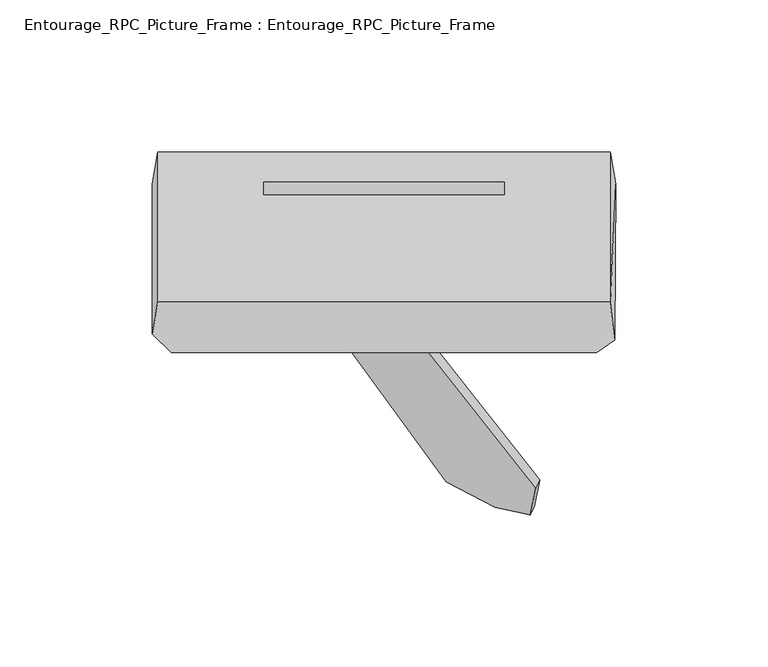
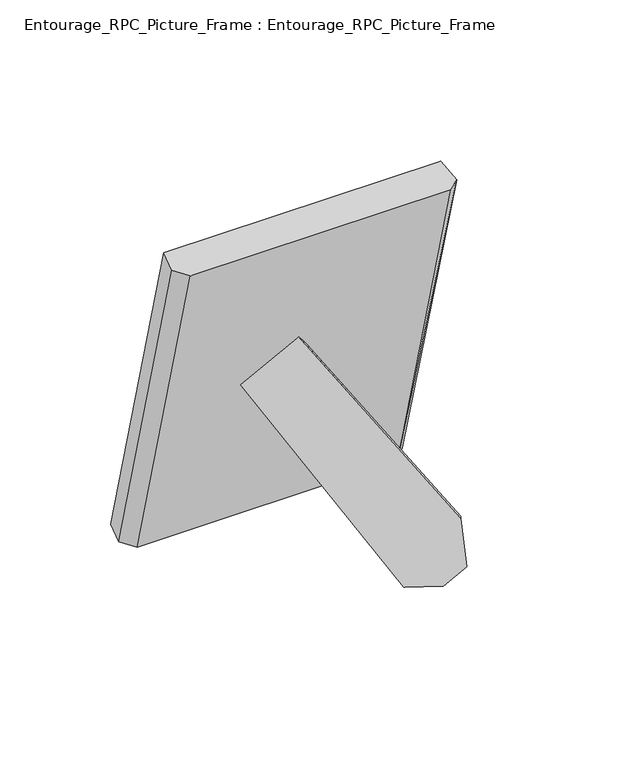
"""IFC4 building model written with IfcOpenShell, lengths in millimetres: proxy geometry, Entourage_RPC_Picture_Frame : Entourage_RPC_Picture_Frame."""

from ifc_helpers import new_model, si_unit, origin, place, context, project, spatial, triangles, source, transform, mapped, element, save


def entourage_rpc_picture_frame_entourage_rpc_picture_frame_0c3f382a(model_context):
    return source(origin(), model_context, "Body", "Tessellation", [
        triangles([(-31.2212752, 21.3179439, 97.8039775), (-3.3552966, 15.6563572, 118.0830721), (49.8722556, -51.6400711, 31.432093), (48.0637995, -60.4893174, 9.6569551), (36.5907671, -58.1576284, 1.3080831), (20.4721357, -49.6588966, 1.1709248), (-29.8344526, 23.9264897, 96.6279682), (-1.9710145, 18.262363, 116.9070629), (51.2565371, -49.0391442, 30.2611684), (49.4455375, -57.8858517, 8.4834904), (37.9725073, -55.5541626, 0.1346183), (21.8564171, -47.0554308, -0.00254), (-74.3118158, 9.430898, 188.4655675), (74.3118158, 9.430898, 188.4655675), (75.7926166, -3.1317793, 185.1001116), (69.8490931, -7.2160464, 184.0053746), (-69.8490931, -7.2160464, 184.0053746), (-76.1990144, -1.082026, 185.6487336), (-74.3118158, 58.7342011, 4.4601824), (74.3118158, 58.7469002, 4.4398626), (76.1990144, 48.2212754, 1.6433587), (69.8490931, 42.0897955, 0.0), (-69.8490931, 42.0897955, 0.0), (-76.1990144, 48.2212754, 1.6433587), (-39.6869853, 19.0954732, 152.4335917), (39.6869853, 19.0954732, 152.436117), (39.6869853, 49.0899451, 40.4972374), (-39.6869853, 49.0899451, 40.4972374), (-39.6869853, 14.7064095, 151.2575824), (39.6869853, 14.7064095, 151.2575824), (39.6869853, 44.7008825, 39.3212327), (-39.6869853, 44.7008825, 39.3212327)], [[1, 2, 8], [1, 8, 7], [2, 3, 9], [2, 9, 8], [3, 4, 10], [3, 10, 9], [4, 5, 11], [4, 11, 10], [5, 6, 12], [5, 12, 11], [6, 1, 7], [6, 7, 12], [1, 3, 2], [6, 3, 1], [6, 4, 3], [5, 4, 6], [7, 8, 9], [12, 7, 9], [12, 9, 10], [11, 12, 10], [15, 17, 16], [14, 17, 15], [13, 17, 14], [18, 17, 13], [21, 22, 23], [20, 21, 23], [19, 20, 23], [24, 19, 23], [23, 22, 16], [16, 17, 23], [20, 19, 27], [27, 19, 28], [14, 25, 13], [26, 25, 14], [14, 20, 27], [27, 26, 14], [28, 19, 13], [13, 25, 28], [29, 32, 28], [28, 25, 29], [30, 29, 25], [25, 26, 30], [31, 30, 26], [26, 27, 31], [32, 31, 27], [27, 28, 32], [31, 32, 29], [30, 31, 29], [14, 15, 21], [14, 21, 20], [15, 16, 22], [15, 22, 21], [17, 18, 24], [17, 24, 23], [18, 13, 19], [18, 19, 24]]),
    ])


if __name__ == "__main__":
    model = new_model("IFC4")
    model_context = context("Model", 3, world=origin())
    ifc_project = project(units=[si_unit("LENGTHUNIT", "METRE", prefix="MILLI")], contexts=[model_context])
    site = spatial("IfcSite", under=ifc_project)
    building = spatial("IfcBuilding", under=site)
    placement = place(None, origin())
    entourage_rpc_picture_frame_entourage_rpc_picture_frame_shape = entourage_rpc_picture_frame_entourage_rpc_picture_frame_0c3f382a(model_context)
    element("IfcBuildingElementProxy", 1, Name="Entourage_RPC_Picture_Frame : Entourage_RPC_Picture_Frame", ObjectType="Entourage_RPC_Picture_Frame : Entourage_RPC_Picture_Frame", at=placement, inside=building, context=model_context, shape_type="MappedRepresentation", body=[
        mapped(entourage_rpc_picture_frame_entourage_rpc_picture_frame_shape, transform((0.0, 0.0, 0.0), x_axis=(1.0, 0.0, 0.0), y_axis=(0.0, 1.0, 0.0), z_axis=(0.0, 0.0, 1.0))),
    ])
    save(model, "model.ifc")

# Revit data of these elements
# Project information
#   Project Status = "Project Status"
#   Client Name = "Revit Project"
#   Project Address = "Enter address here"
#   Project Name = "Two Storey Residence"
#   Project Number = "P.01"
# Type "Entourage_RPC_Picture_Frame : Entourage_RPC_Picture_Frame"
#   built-in parameter 1005198 = "{2, 15},{39, RPC-16-8M5E-0H3T-F0AH-3U0K-JLQ7-G28B-AU},{1, 0},{1, 0},{2, 19},{1, 8},{5, Color},{1, 0},{1, 0},{3, 0.8},{3, 0.8},{3, 0.8},{1, 8},{7, BBoxMin},{1, 0},{1, 0},{1, 0},{1, 0},{1, 0},{1, 8},{7, BBoxMax},{1, 0},{1, 0},{1, 0},{1, 0},{1, 0},{2, 11},{9, RPCTypeId},{1, 0},{1, 0},{39, RPC-16-8M5E-0H3T-F0AH-3U0K-JLQ7-G28B-AU},{1, 6},{14, RPCPlantHeight},{1, 0},{1, 0},{8, 0.624409},{2, 11},{7, keyword},{1, 0},{1, 0},{33, :RPCs:Office Clutter:Geometry:RPC},{2, 11},{8, category},{1, 0},{1, 0},{14, Office Clutter},{2, 11},{12, LocalizedUID},{1, 0},{1, 0},{13, Picture Frame},{2, 14},{6, Height},{1, 0},{1, 0},{8, 0.624409},{1, 2},{16, Cast Reflections},{1, 0},{1, 0},{1, 0},{1, 2},{8, Portrait},{1, 0},{1, 0},{1, 1},{1, 2},{5, Stand},{1, 0},{1, 0},{1, 1},{2, 11},{10, RPCL_Frame},{1, 0},{1, 0},{5, Frame},{1, 4},{14, Frame Material},{1, 0},{1, 0},{1, 0},{2, 11},{12, RPCL_Picture},{1, 0},{1, 0},{7, Picture},{2, 11},{15, Picture Preview},{1, 0},{1, 0},{65, __RPC:/object data/textures/object/Photo/Photo0/textures/Portrait},{2, 11},{17, i_Picture Preview},{1, 0},{1, 0},{0, },{1, 2},{18, Use Custom Picture},{1, 0},{1, 0},{1, 0},{2, 11},{17, Picture File Name},{1, 0},{1, 0},{0, },{21, assetlibrary_base.fbx},{1, 5},"
#   built-in parameter 1005195 = "RPC-16-8M5E-0H3T-F0AH-3U0K-JLQ7-G28B-AU"
#   Height = 0
